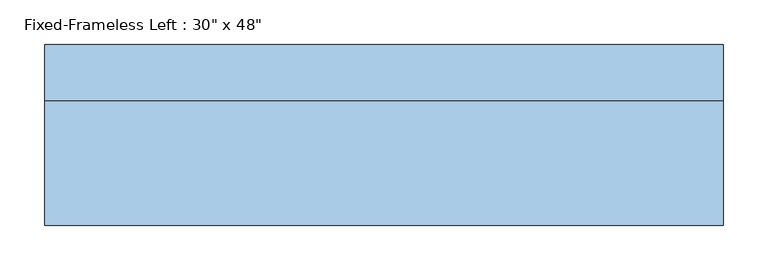
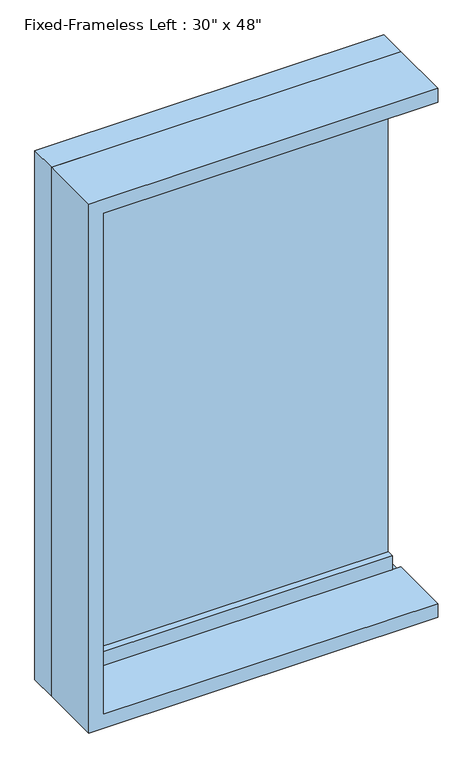
"""IFC4 building model written with IfcOpenShell, lengths in millimetres: window geometry."""

import ifcopenshell
import ifcopenshell.guid

model = None  # the IFC model being written
_history = None  # IfcOwnerHistory: only IFC2X3 demands one
_inside = {}  # id of a spatial element -> (the spatial element, [elements in it])
_under = {}  # id of a project, library or spatial element -> (it, [spatial elements below it])
_declared = {}  # id of a project -> (the project, [libraries it declares])
_typed = {}  # id of a type object -> (the type object, [elements of that type])
_made_of = {}  # id of a material, layer set ... -> (it, [elements and type objects made of it])


def new_model(schema):
    """Start an empty IFC model of exactly this schema.

    Asked for "IFC4X3", IfcOpenShell would pick the latest addendum, in which some entities
    have other attributes; the version numbers below select the first issue.
    IFC2X3 requires an IfcOwnerHistory on every rooted entity: one is made here for all.
    """
    global model, _history
    if schema == "IFC4X3":
        model = ifcopenshell.file(schema_version=(4, 3, 0, 0))
    else:
        model = ifcopenshell.file(schema=schema)
    _inside.clear()
    _under.clear()
    _declared.clear()
    _typed.clear()
    _made_of.clear()
    _history = None
    if model.schema == "IFC2X3":
        org = make("IfcOrganization", Name="unknown")
        user = make(
            "IfcPersonAndOrganization",
            ThePerson=make("IfcPerson", FamilyName="unknown"),
            TheOrganization=org,
        )
        app = make(
            "IfcApplication",
            ApplicationDeveloper=org,
            Version="unknown",
            ApplicationFullName="unknown",
            ApplicationIdentifier="unknown",
        )
        _history = make(
            "IfcOwnerHistory",
            OwningUser=user,
            OwningApplication=app,
            ChangeAction="ADDED",
            CreationDate=0,
        )
    return model


def make(cls, **values):
    """One entity of the class cls with the attributes given. An attribute that is None is left unset."""
    return model.create_entity(
        cls, **{name: value for name, value in values.items() if value is not None}
    )


def rooted(cls, **values):
    """An entity with a GlobalId (a new one), such as an element, a storey or a relation."""
    return make(cls, GlobalId=ifcopenshell.guid.new(), OwnerHistory=_history, **values)


def si_unit(unit_type, name, prefix=None):
    """IfcSIUnit, for example si_unit("LENGTHUNIT", "METRE", prefix="MILLI")."""
    return make("IfcSIUnit", UnitType=unit_type, Prefix=prefix, Name=name)


def assignment(units):
    """IfcUnitAssignment: the units of a project."""
    return None if units is None else make("IfcUnitAssignment", Units=units)


def point(xyz):
    """IfcCartesianPoint."""
    return None if xyz is None else make("IfcCartesianPoint", Coordinates=xyz)


def direction(xyz):
    """IfcDirection."""
    return None if xyz is None else make("IfcDirection", DirectionRatios=xyz)


def frame(location, z_axis=None, x_axis=None):
    """IfcAxis2Placement3D, a coordinate frame: its origin and axes. An axis left out is left unset."""
    return make(
        "IfcAxis2Placement3D",
        Location=point(location),
        Axis=direction(z_axis),
        RefDirection=direction(x_axis),
    )


def origin():
    """The frame at (0, 0, 0) with its axes left unset."""
    return frame((0.0, 0.0, 0.0))


def place(relative_to, where):
    """IfcLocalPlacement: puts the frame where relative to a parent placement (None: the world)."""
    return make(
        "IfcLocalPlacement", PlacementRelTo=relative_to, RelativePlacement=where
    )


def context(
    kind, dimensions, precision=None, world=None, true_north=None, identifier=None
):
    """IfcGeometricRepresentationContext, for example the 3D "Model" context."""
    return make(
        "IfcGeometricRepresentationContext",
        ContextIdentifier=identifier,
        ContextType=kind,
        CoordinateSpaceDimension=dimensions,
        Precision=precision,
        WorldCoordinateSystem=world,
        TrueNorth=true_north,
    )


def project(units=None, contexts=None):
    """IfcProject with its units and contexts."""
    return rooted(
        "IfcProject",
        Name="project",
        RepresentationContexts=contexts,
        UnitsInContext=assignment(units),
    )


def spatial(cls, under=None, at=None, **own):
    """A site, building, storey or space (cls), placed at a placement, below another one or the project."""
    s = rooted(cls, ObjectPlacement=at, **own)
    if under is not None:
        _under.setdefault(under.id(), (under, []))[1].append(s)
    return s


def polyline(points):
    """IfcPolyline through the points."""
    return make("IfcPolyline", Points=[point(p) for p in points])


def outline(outer, holes=None, kind="AREA"):
    """IfcArbitraryClosedProfileDef: a profile drawn as a closed curve; with holes, ...WithVoids."""
    if holes is None:
        return make("IfcArbitraryClosedProfileDef", ProfileType=kind, OuterCurve=outer)
    return make(
        "IfcArbitraryProfileDefWithVoids",
        ProfileType=kind,
        OuterCurve=outer,
        InnerCurves=holes,
    )


def extrude(swept, where, along, depth):
    """IfcExtrudedAreaSolid: the profile swept, set in the frame where, extruded along a direction by depth."""
    return make(
        "IfcExtrudedAreaSolid",
        SweptArea=swept,
        Position=where,
        ExtrudedDirection=direction(along),
        Depth=depth,
    )


def shape(context_of_items, identifier, shape_type, items):
    """IfcShapeRepresentation: the items that make up one representation, for example the "Body"."""
    return make(
        "IfcShapeRepresentation",
        ContextOfItems=context_of_items,
        RepresentationIdentifier=identifier,
        RepresentationType=shape_type,
        Items=items,
    )


def source(mapping_origin, context_of_items, identifier, shape_type, items):
    """IfcRepresentationMap: a shape defined once, which mapped items show again and again."""
    return make(
        "IfcRepresentationMap",
        MappingOrigin=mapping_origin,
        MappedRepresentation=shape(context_of_items, identifier, shape_type, items),
    )


def transform(
    local_origin,
    x_axis=None,
    y_axis=None,
    z_axis=None,
    scale=None,
    scale2=None,
    scale3=None,
    uniform=True,
):
    """IfcCartesianTransformationOperator3D, or its non-uniform kind. x_axis, y_axis, z_axis: its Axis1, 2, 3."""
    if uniform:
        return make(
            "IfcCartesianTransformationOperator3D",
            Axis1=direction(x_axis),
            Axis2=direction(y_axis),
            LocalOrigin=point(local_origin),
            Scale=scale,
            Axis3=direction(z_axis),
        )
    return make(
        "IfcCartesianTransformationOperator3DnonUniform",
        Axis1=direction(x_axis),
        Axis2=direction(y_axis),
        LocalOrigin=point(local_origin),
        Scale=scale,
        Axis3=direction(z_axis),
        Scale2=scale2,
        Scale3=scale3,
    )


def mapped(mapping_source, mapping_target):
    """IfcMappedItem: shows the shape of a source again, moved by a transform."""
    return make(
        "IfcMappedItem", MappingSource=mapping_source, MappingTarget=mapping_target
    )


def made_of(thing, what):
    """Note that an element or type object is made of a material, layer set ...; save() writes the relation."""
    if what is not None:
        _made_of.setdefault(what.id(), (what, []))[1].append(thing)
    return thing


def element(
    cls,
    number,
    at=None,
    inside=None,
    cuts=None,
    type_object=None,
    material=None,
    context=None,
    identifier="Body",
    shape_type=None,
    held_by="IfcProductDefinitionShape",
    body=None,
    shapes=None,
    **own,
):
    """One element of the class cls, such as IfcWall. Its Tag is "e" and its number.

    at: its placement. inside: the storey or other place that contains it. cuts: it is an
    opening in that element (IfcRelVoidsElement). A single representation is given by context,
    identifier, shape_type and body (its items); several are given by shapes. held_by: the class
    of the entity that holds the representations. save() writes the other relations.
    """
    e = rooted(cls, Tag="e%d" % number, ObjectPlacement=at, **own)
    if body is not None:
        shapes = [shape(context, identifier, shape_type, body)]
    if shapes is not None:
        e.Representation = make(held_by, Representations=shapes)
    if inside is not None:
        _inside.setdefault(inside.id(), (inside, []))[1].append(e)
    if cuts is not None:
        rooted(
            "IfcRelVoidsElement", RelatingBuildingElement=cuts, RelatedOpeningElement=e
        )
    if type_object is not None:
        _typed.setdefault(type_object.id(), (type_object, []))[1].append(e)
    return made_of(e, material)


def aggregate(whole, parts):
    """IfcRelAggregates: a whole, such as a stair, and the parts it consists of."""
    return rooted("IfcRelAggregates", RelatingObject=whole, RelatedObjects=parts)


def save(model, path):
    """Write the relations noted so far, then the file.

    IfcRelAggregates (storeys below a building ...), IfcRelContainedInSpatialStructure (elements
    in a storey), IfcRelDefinesByType, IfcRelAssociatesMaterial and IfcRelDeclares: one each for
    every whole, place, type object, material and project.
    """
    for whole, parts in _under.values():
        aggregate(whole, parts)
    for where, things in _inside.values():
        rooted(
            "IfcRelContainedInSpatialStructure",
            RelatedElements=things,
            RelatingStructure=where,
        )
    for kind, things in _typed.values():
        rooted("IfcRelDefinesByType", RelatedObjects=things, RelatingType=kind)
    for what, things in _made_of.values():
        rooted("IfcRelAssociatesMaterial", RelatedObjects=things, RelatingMaterial=what)
    for by, libraries in _declared.values():
        rooted("IfcRelDeclares", RelatingContext=by, RelatedDefinitions=libraries)
    model.write(path)


def window_e404f2f7(model_context):
    return source(origin(), model_context, "Body", "SweptSolid", [
        extrude(outline(polyline([(323.85, 53.975), (-355.6, 53.975), (-355.6, 66.675), (323.85, 66.675), (323.85, 53.975)])), frame((0.0, 0.0, 977.9), z_axis=(0.0, 0.0, 1.0), x_axis=(1.0, 0.0, 0.0)), (0.0, 0.0, 1.0), 1092.2),
        extrude(outline(polyline([(2114.55, -400.05), (933.45, -400.05), (933.45, 323.85), (977.9, 323.85), (977.9, -355.6), (2070.1, -355.6), (2070.1, 323.85), (2114.55, 323.85), (2114.55, -400.05)])), frame((0.0, 38.1, 0.0), z_axis=(0.0, 1.0, 0.0), x_axis=(0.0, 0.0, 1.0)), (0.0, 0.0, 1.0), 44.45),
        extrude(outline(polyline([(2133.6, -419.1), (914.4, -419.1), (914.4, 342.9), (946.15, 342.9), (946.15, -387.35), (2101.85, -387.35), (2101.85, 342.9), (2133.6, 342.9), (2133.6, -419.1)])), frame((0.0, -101.6, 0.0), z_axis=(0.0, 1.0, 0.0), x_axis=(0.0, 0.0, 1.0)), (0.0, 0.0, 1.0), 139.7),
        extrude(outline(polyline([(2133.6, 342.9), (2133.6, -419.1), (914.4, -419.1), (914.4, 342.9), (933.45, 342.9), (933.45, -400.05), (2114.55, -400.05), (2114.55, 342.9), (2133.6, 342.9)])), frame((0.0, 38.1, 0.0), z_axis=(0.0, 1.0, 0.0), x_axis=(0.0, 0.0, 1.0)), (0.0, 0.0, 1.0), 63.5),
    ])


if __name__ == "__main__":
    model = new_model("IFC4")
    model_context = context("Model", 3, world=origin())
    ifc_project = project(units=[si_unit("LENGTHUNIT", "METRE", prefix="MILLI")], contexts=[model_context])
    site = spatial("IfcSite", under=ifc_project)
    building = spatial("IfcBuilding", under=site)
    placement = place(None, origin())
    window_shape = window_e404f2f7(model_context)
    element("IfcWindow", 1, ObjectType="Fixed-Frameless Left : 30\" x 48\"", at=placement, inside=building, context=model_context, shape_type="MappedRepresentation", body=[
        mapped(window_shape, transform((0.0, 0.0, 0.0), x_axis=(1.0, 0.0, 0.0), y_axis=(0.0, 1.0, 0.0), z_axis=(0.0, 0.0, 1.0))),
    ])
    save(model, "model.ifc")

# Revit data of these elements
# Project information
#   Project Issue Date = "Issue Date"
#   Project Status = "Project Status"
#   Client Name = "Owner"
#   Project Address = "Enter address here"
#   Project Name = "Project Name"
#   Project Number = "Project Number"
#   SR Document GUID = "4bc87e05-88e2-428e-9b18-4d898ac90ae1"
# Type "Fixed-Frameless Left : 30\" x 48\""
#   Type Mark = "75"
#   Assembly Code = "B2020100"
#   Height = 4' - 0"
#   Default Sill Height = 3' - 0"
#   Width = 2' - 6"
#   Window Inset = 0' - 0 3/4"
#   Glass Pane Material = Glass
#   Sash Material = Sash
#   Wall Closure = (empty or 0)
# Element 1 (IfcWindow, "Fixed-Frameless Left : 30\" x 48\"")
#   Materials on its faces: "Sash", "Glass"
# Materials
#   "Glass": class "Glass", colour RGB 0 128 192, transparency 0.75
#   "Sash": class "Wood", colour RGB 224 178 126, transparency 0
